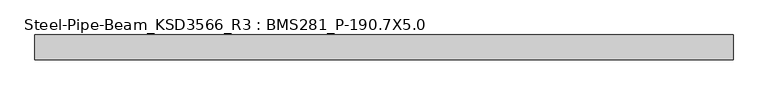
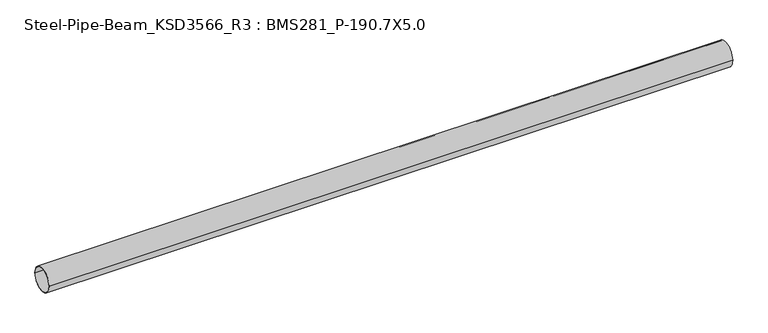
"""IFC4 building model written with IfcOpenShell, lengths in millimetres: member geometry, Steel-Pipe-Beam_KSD3566_R3 : BMS281_P-190.7X5.0."""

from ifc_helpers import new_model, si_unit, point, frame, origin, origin_2d, place, context, project, spatial, circle_curve, trimmed, segment, composite_curve, outline, extrude, source, transform, mapped, element, save


def steel_pipe_beam_ksd3566_r3_bms281_p_190_7x5_0_e894cb2c(model_context):
    return source(origin(), model_context, "Body", "SweptSolid", [
        extrude(outline(composite_curve([segment(trimmed(circle_curve(origin_2d(), 95.35), [point((-95.35, 0.0))], [point((95.35, 0.0))], False, "CARTESIAN"), True, "CONTINUOUS"), segment(trimmed(circle_curve(origin_2d(), 95.35), [point((95.35, 0.0))], [point((-95.35, 0.0))], False, "CARTESIAN"), True, "CONTINUOUS")], self_intersect=False), holes=[composite_curve([segment(trimmed(circle_curve(origin_2d(), 90.35), [point((90.35, 0.0))], [point((-90.35, 0.0))], True, "CARTESIAN"), True, "CONTINUOUS"), segment(trimmed(circle_curve(origin_2d(), 90.35), [point((-90.35, 0.0))], [point((90.35, 0.0))], True, "CARTESIAN"), True, "CONTINUOUS")], self_intersect=False)]), frame((-2577.3899291, 0.0, 0.0), z_axis=(1.0, 0.0, 0.0), x_axis=(0.0, 1.0, 0.0)), (0.0, 0.0, 1.0), 5329.8345025),
    ])


if __name__ == "__main__":
    model = new_model("IFC4")
    model_context = context("Model", 3, world=origin())
    ifc_project = project(units=[si_unit("LENGTHUNIT", "METRE", prefix="MILLI")], contexts=[model_context])
    site = spatial("IfcSite", under=ifc_project)
    building = spatial("IfcBuilding", under=site)
    placement = place(None, origin())
    steel_pipe_beam_ksd3566_r3_bms281_p_190_7x5_0_shape = steel_pipe_beam_ksd3566_r3_bms281_p_190_7x5_0_e894cb2c(model_context)
    element("IfcMember", 1, ObjectType="Steel-Pipe-Beam_KSD3566_R3 : BMS281_P-190.7X5.0", at=placement, inside=building, context=model_context, shape_type="MappedRepresentation", body=[
        mapped(steel_pipe_beam_ksd3566_r3_bms281_p_190_7x5_0_shape, transform((0.0, 0.0, 0.0), x_axis=(1.0, 0.0, 0.0), y_axis=(0.0, 1.0, 0.0), z_axis=(0.0, 0.0, 1.0))),
    ])
    save(model, "model.ifc")

# Revit data of these elements
# Type "Steel-Pipe-Beam_KSD3566_R3 : BMS281_P-190.7X5.0"
#   Keynote = "P-190.7X5.0"
#   SteelWeight = "Light"
#   t = 0.0050 m
#   Surface Area = 0.599102 m²/m
#   Section Area = 29.1697 cm²
#   Mass per Unit Length = 22.8982 kg/m
#   Length [instance default] = 1.5000 m
#   D = 0.1907 m
#   hec_material4 [instance default] = none
#   hec_material3 [instance default] = none
#   hec_material2 [instance default] = none
#   hec_material1 [instance default] = none
#   Structural Material [instance default] = Steel, 45-345
#   Assembly Code = ""
# Element 1 (IfcMember, "Steel-Pipe-Beam_KSD3566_R3 : BMS281_P-190.7X5.0")
#   Structural Material = none
# Materials
#   "Steel, 45-345": class "Metal", colour RGB 189 187 185, transparency 0, Description = "Steel 345 MPa", Cost = 0
